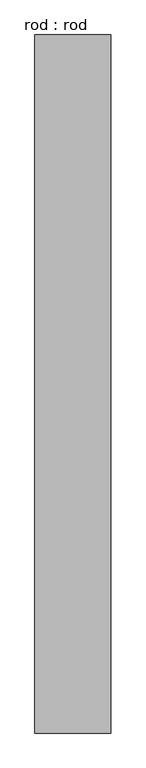
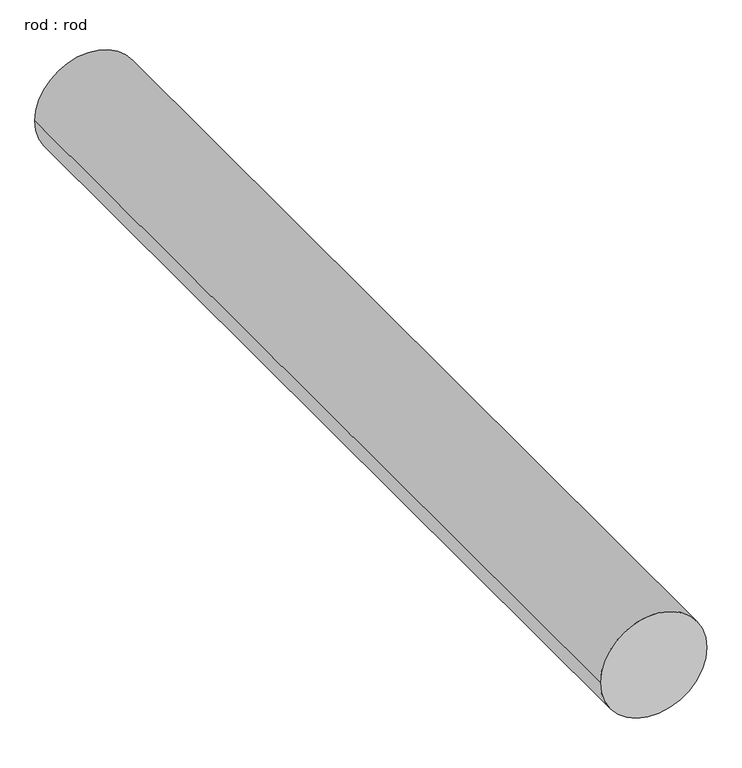
"""IFC4 building model written with IfcOpenShell, lengths in millimetres: proxy geometry, rod : rod."""

from ifc_helpers import new_model, si_unit, point, frame, frame_2d, origin, place, context, project, spatial, circle_curve, trimmed, segment, composite_curve, outline, extrude, source, transform, mapped, element, save


def rod_rod_c52567e6(model_context):
    return source(origin(), model_context, "Body", "SweptSolid", [
        extrude(outline(composite_curve([segment(trimmed(circle_curve(frame_2d((0.0108462, 0.0)), 200.0), [point((0.0108462, 200.0))], [point((0.0108462, -200.0))], False, "CARTESIAN"), True, "CONTINUOUS"), segment(trimmed(circle_curve(frame_2d((0.0108462, 0.0)), 200.0), [point((0.0108462, -200.0))], [point((0.0108462, 200.0))], False, "CARTESIAN"), True, "CONTINUOUS")], self_intersect=False)), frame((0.0, 2256.4943574, 0.0), z_axis=(0.0, 1.0, 0.0), x_axis=(0.0, 0.0, 1.0)), (0.0, 0.0, 1.0), 3672.4685159),
    ])


if __name__ == "__main__":
    model = new_model("IFC4")
    model_context = context("Model", 3, world=origin())
    ifc_project = project(units=[si_unit("LENGTHUNIT", "METRE", prefix="MILLI")], contexts=[model_context])
    site = spatial("IfcSite", under=ifc_project)
    building = spatial("IfcBuilding", under=site)
    placement = place(None, origin())
    rod_rod_shape = rod_rod_c52567e6(model_context)
    element("IfcBuildingElementProxy", 1, Name="rod : rod", ObjectType="rod : rod", at=placement, inside=building, context=model_context, shape_type="MappedRepresentation", body=[
        mapped(rod_rod_shape, transform((0.0, 0.0, 0.0), x_axis=(1.0, 0.0, 0.0), y_axis=(0.0, 1.0, 0.0), z_axis=(0.0, 0.0, 1.0))),
    ])
    save(model, "model.ifc")

# Revit data of these elements
# Type "rod : rod"
#   Default Elevation = 0
